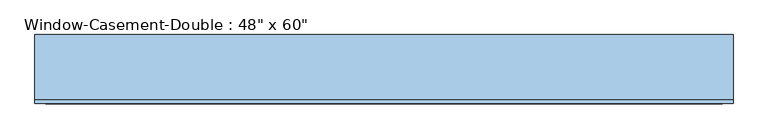
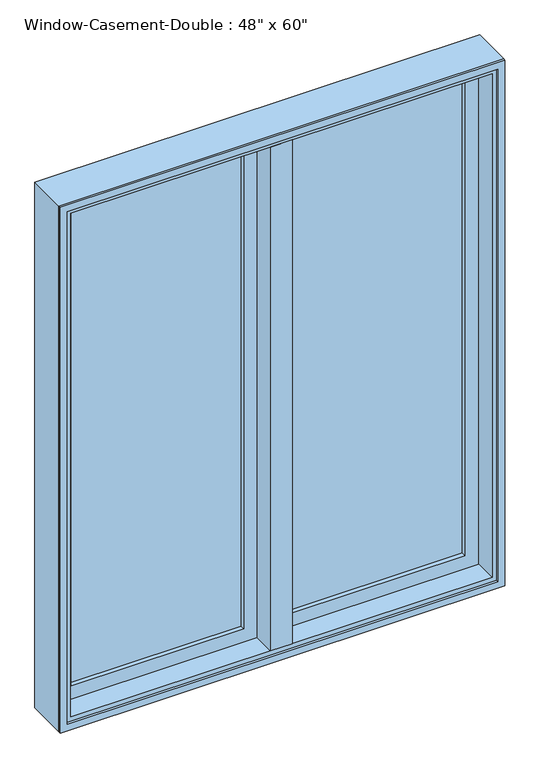
"""IFC4 building model written with IfcOpenShell, lengths in millimetres: window geometry."""

from ifc_helpers import new_model, si_unit, frame, origin, place, context, project, spatial, polyline, outline, extrude, faceted_brep, source, transform, mapped, element, save


def window_6b856993(model_context):
    return source(origin(), model_context, "Body", "SolidModel", [
        faceted_brep([(9.525, 69.85, 2425.7), (-9.525, 69.85, 2425.7), (-9.525, 19.05, 2425.7), (9.525, 19.05, 2425.7), (9.525, 69.85, 927.1), (9.525, 19.05, 927.1), (-9.525, 19.05, 927.1), (-9.525, 69.85, 927.1), (-9.525, 19.05, 946.15), (-9.525, 19.05, 2406.65), (-30.1625, 19.05, 946.15), (-30.1625, 19.05, 2406.65), (-30.1625, -44.45, 946.15), (-30.1625, -44.45, 2406.65), (30.1625, -44.45, 946.15), (30.1625, -44.45, 2406.65), (30.1625, 19.05, 946.15), (30.1625, 19.05, 2406.65), (9.525, 19.05, 946.15), (9.525, 19.05, 2406.65)], [[[0, 1, 2, 3]], [[4, 5, 6, 7]], [[1, 0, 4, 7]], [[2, 1, 7, 6, 8, 9]], [[9, 8, 10, 11]], [[11, 10, 12, 13]], [[13, 12, 14, 15]], [[15, 14, 16, 17]], [[17, 16, 18, 19]], [[0, 3, 19, 18, 5, 4]], [[18, 8, 6, 5]], [[9, 19, 3, 2]], [[8, 18, 16, 14, 12, 10]], [[19, 9, 11, 13, 15, 17]]]),
        extrude(outline(polyline([(-66.675, 50.8), (-66.675, 44.45), (-539.75, 44.45), (-539.75, 50.8), (-66.675, 50.8)])), frame((0.0, 0.0, 984.25), z_axis=(0.0, 0.0, 1.0), x_axis=(1.0, 0.0, 0.0)), (0.0, 0.0, 1.0), 1384.3),
        extrude(outline(polyline([(-539.75, 31.75), (-539.75, 38.1), (-66.675, 38.1), (-66.675, 31.75), (-539.75, 31.75)])), frame((0.0, 0.0, 984.25), z_axis=(0.0, 0.0, 1.0), x_axis=(1.0, 0.0, 0.0)), (0.0, 0.0, 1.0), 1384.3),
        extrude(outline(polyline([(539.75, 50.8), (539.75, 44.45), (66.675, 44.45), (66.675, 50.8), (539.75, 50.8)])), frame((0.0, 0.0, 984.25), z_axis=(0.0, 0.0, 1.0), x_axis=(1.0, 0.0, 0.0)), (0.0, 0.0, 1.0), 1384.3),
        extrude(outline(polyline([(66.675, 31.75), (66.675, 38.1), (539.75, 38.1), (539.75, 31.75), (66.675, 31.75)])), frame((0.0, 0.0, 984.25), z_axis=(0.0, 0.0, 1.0), x_axis=(1.0, 0.0, 0.0)), (0.0, 0.0, 1.0), 1384.3),
        extrude(outline(polyline([(2425.7, -596.9), (927.1, -596.9), (927.1, -9.525), (2425.7, -9.525), (2425.7, -596.9)]), holes=[polyline([(2368.55, -66.675), (984.25, -66.675), (984.25, -539.75), (2368.55, -539.75), (2368.55, -66.675)])]), frame((0.0, 19.05, 0.0), z_axis=(0.0, 1.0, 0.0), x_axis=(0.0, 0.0, 1.0)), (0.0, 0.0, 1.0), 44.45),
        extrude(outline(polyline([(927.1, 596.9), (2425.7, 596.9), (2425.7, 9.525), (927.1, 9.525), (927.1, 596.9)]), holes=[polyline([(984.25, 66.675), (2368.55, 66.675), (2368.55, 539.75), (984.25, 539.75), (984.25, 66.675)])]), frame((0.0, 19.05, 0.0), z_axis=(0.0, 1.0, 0.0), x_axis=(0.0, 0.0, 1.0)), (0.0, 0.0, 1.0), 44.45),
        extrude(outline(polyline([(2438.4, -609.6), (914.4, -609.6), (914.4, 609.6), (2438.4, 609.6), (2438.4, -609.6)]), holes=[polyline([(2419.35, 590.55), (933.45, 590.55), (933.45, -590.55), (2419.35, -590.55), (2419.35, 590.55)])]), frame((0.0, -50.8, 0.0), z_axis=(0.0, 1.0, 0.0), x_axis=(0.0, 0.0, 1.0)), (0.0, 0.0, 1.0), 6.35),
        faceted_brep([(577.85, 19.05, 2406.65), (577.85, -44.45, 2406.65), (-577.85, -44.45, 2406.65), (-577.85, 19.05, 2406.65), (596.9, 69.85, 2425.7), (596.9, 19.05, 2425.7), (-596.9, 19.05, 2425.7), (-596.9, 69.85, 2425.7), (609.6, -44.45, 2438.4), (609.6, 69.85, 2438.4), (-609.6, 69.85, 2438.4), (-609.6, -44.45, 2438.4), (-577.85, -44.45, 946.15), (-577.85, 19.05, 946.15), (-596.9, 19.05, 927.1), (-596.9, 69.85, 927.1), (-609.6, 69.85, 914.4), (-609.6, -44.45, 914.4), (577.85, -44.45, 946.15), (577.85, 19.05, 946.15), (596.9, 19.05, 927.1), (596.9, 69.85, 927.1), (609.6, 69.85, 914.4), (609.6, -44.45, 914.4)], [[[0, 1, 2, 3]], [[4, 5, 6, 7]], [[8, 9, 10, 11]], [[3, 2, 12, 13]], [[7, 6, 14, 15]], [[11, 10, 16, 17]], [[13, 12, 18, 19]], [[15, 14, 20, 21]], [[17, 16, 22, 23]], [[11, 17, 23, 8], [1, 18, 12, 2]], [[19, 18, 1, 0]], [[5, 20, 14, 6], [3, 13, 19, 0]], [[21, 20, 5, 4]], [[23, 22, 9, 8]], [[9, 22, 16, 10], [7, 15, 21, 4]]]),
    ])


if __name__ == "__main__":
    model = new_model("IFC4")
    model_context = context("Model", 3, world=origin())
    ifc_project = project(units=[si_unit("LENGTHUNIT", "METRE", prefix="MILLI")], contexts=[model_context])
    site = spatial("IfcSite", under=ifc_project)
    building = spatial("IfcBuilding", under=site)
    placement = place(None, origin())
    window_shape = window_6b856993(model_context)
    element("IfcWindow", 1, ObjectType="Window-Casement-Double : 48\" x 60\"", at=placement, inside=building, context=model_context, shape_type="MappedRepresentation", body=[
        mapped(window_shape, transform((0.0, 0.0, 0.0), x_axis=(1.0, 0.0, 0.0), y_axis=(0.0, 1.0, 0.0), z_axis=(0.0, 0.0, 1.0))),
    ])
    save(model, "model.ifc")

# Revit data of these elements
# Type "Window-Casement-Double : 48\" x 60\""
#   Type Mark = "61"
#   Fire Rating = "0.5h"
#   Assembly Code = "B2020100"
#   Analytic Construction = "Double glazing - domestic"
#   Frame Extension [instance default] = 0' - 0 1/4"
#   Window Inset [instance default] = 0' - 0"
#   Wall Thickness [instance default] = 0' - 6"
#   Interior Wall Closure [instance default] = 0' - 2 1/4"
#   Half Width = 2' - 0"
#   Visual Light Transmittance = 0.81
#   Thermal Resistance (R) = 1.8146 (h·ft²·°F)/BTU
#   Solar Heat Gain Coefficient = 0.76
#   Rough Width = 4' - 0 1/2"
#   Rough Height = 5' - 0 1/2"
#   Height = 5' - 0"
#   Heat Transfer Coefficient (U) = 0.5511 BTU/(h·ft²·°F)
#   Exterior Wall Closure [instance default] = 0' - 1 1/4"
#   Extension Jamb [instance default] = 0' - 2 1/4"
#   Default Sill Height = 3' - 0"
#   Width = 4' - 0"
#   Define Thermal Properties by = 0
#   Muntin Visibility = yes
#   Interior Trim Visibility [instance default] = yes
#   Exterior Trim Visibility [instance default] = yes
#   Extension Jamb Visibility [instance default] = yes
#   Interior Trim Material = Wood - Stained
#   Muntin Pattern = Muntin Pattern_2x2 : Muntin Pattern_2x2
#   Interior Trim = Trim-Window-Interior-Flat : Picture Frame
#   Interior Frame Material = Wood - Stained
#   Glass Panel Material = Glass
#   Exterior Trim Material = Clad - White
#   Exterior Trim = Trim-Window-Exterior-Flat : with Sill
#   Exterior Frame Material = Clad - White
#   Wall Closure = (empty or 0)
# Element 1 (IfcWindow, "Window-Casement-Double : 48\" x 60\"")
#   Wall Thickness = 0' - 4"
#   Extension Jamb = 0' - 0 1/4"
#   Materials on its faces: "Wood - Stained", "Glass", "Clad - White"
# Materials
#   "Wood - Stained": class "Wood", colour RGB 224 178 126, transparency 0, Cost = 0
#   "Glass": class "Glass", colour RGB 236 240 239, transparency 0.5, Description = "Soda Lime Glass", Cost = 0
#   "Clad - White": class "Wood", colour RGB 216 216 204, transparency 0, Cost = 0
